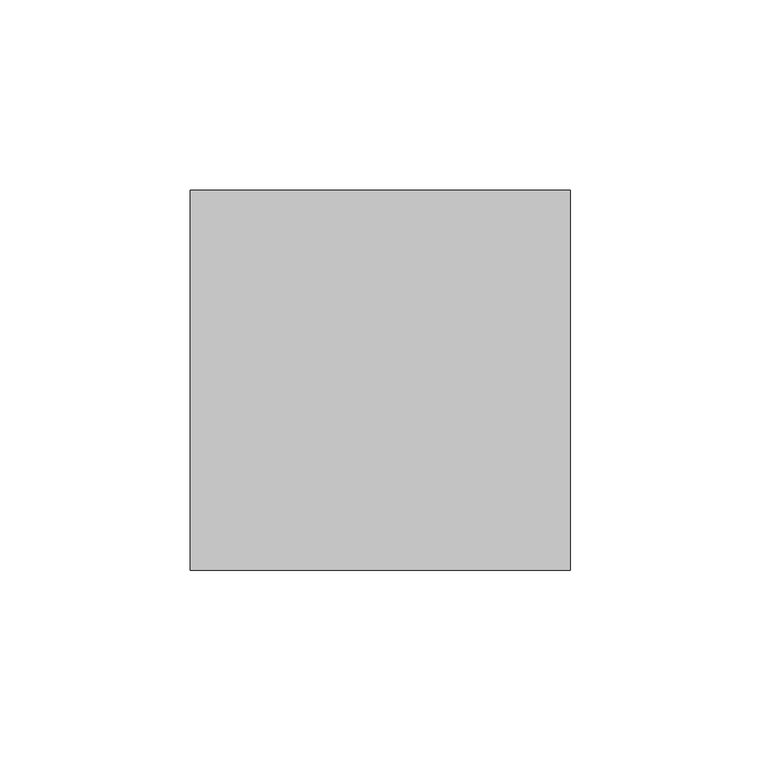
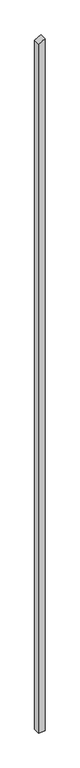
"""IFC4 building model written with IfcOpenShell, lengths in millimetres: column geometry, Holzstütze 159706 : Holzstütze 159706."""

import ifcopenshell
import ifcopenshell.guid

model = None  # the IFC model being written
_history = None  # IfcOwnerHistory: only IFC2X3 demands one
_inside = {}  # id of a spatial element -> (the spatial element, [elements in it])
_under = {}  # id of a project, library or spatial element -> (it, [spatial elements below it])
_declared = {}  # id of a project -> (the project, [libraries it declares])
_typed = {}  # id of a type object -> (the type object, [elements of that type])
_made_of = {}  # id of a material, layer set ... -> (it, [elements and type objects made of it])


def new_model(schema):
    """Start an empty IFC model of exactly this schema.

    Asked for "IFC4X3", IfcOpenShell would pick the latest addendum, in which some entities
    have other attributes; the version numbers below select the first issue.
    IFC2X3 requires an IfcOwnerHistory on every rooted entity: one is made here for all.
    """
    global model, _history
    if schema == "IFC4X3":
        model = ifcopenshell.file(schema_version=(4, 3, 0, 0))
    else:
        model = ifcopenshell.file(schema=schema)
    _inside.clear()
    _under.clear()
    _declared.clear()
    _typed.clear()
    _made_of.clear()
    _history = None
    if model.schema == "IFC2X3":
        org = make("IfcOrganization", Name="unknown")
        user = make(
            "IfcPersonAndOrganization",
            ThePerson=make("IfcPerson", FamilyName="unknown"),
            TheOrganization=org,
        )
        app = make(
            "IfcApplication",
            ApplicationDeveloper=org,
            Version="unknown",
            ApplicationFullName="unknown",
            ApplicationIdentifier="unknown",
        )
        _history = make(
            "IfcOwnerHistory",
            OwningUser=user,
            OwningApplication=app,
            ChangeAction="ADDED",
            CreationDate=0,
        )
    return model


def make(cls, **values):
    """One entity of the class cls with the attributes given. An attribute that is None is left unset."""
    return model.create_entity(
        cls, **{name: value for name, value in values.items() if value is not None}
    )


def rooted(cls, **values):
    """An entity with a GlobalId (a new one), such as an element, a storey or a relation."""
    return make(cls, GlobalId=ifcopenshell.guid.new(), OwnerHistory=_history, **values)


def si_unit(unit_type, name, prefix=None):
    """IfcSIUnit, for example si_unit("LENGTHUNIT", "METRE", prefix="MILLI")."""
    return make("IfcSIUnit", UnitType=unit_type, Prefix=prefix, Name=name)


def assignment(units):
    """IfcUnitAssignment: the units of a project."""
    return None if units is None else make("IfcUnitAssignment", Units=units)


def point(xyz):
    """IfcCartesianPoint."""
    return None if xyz is None else make("IfcCartesianPoint", Coordinates=xyz)


def direction(xyz):
    """IfcDirection."""
    return None if xyz is None else make("IfcDirection", DirectionRatios=xyz)


def frame(location, z_axis=None, x_axis=None):
    """IfcAxis2Placement3D, a coordinate frame: its origin and axes. An axis left out is left unset."""
    return make(
        "IfcAxis2Placement3D",
        Location=point(location),
        Axis=direction(z_axis),
        RefDirection=direction(x_axis),
    )


def origin():
    """The frame at (0, 0, 0) with its axes left unset."""
    return frame((0.0, 0.0, 0.0))


def place(relative_to, where):
    """IfcLocalPlacement: puts the frame where relative to a parent placement (None: the world)."""
    return make(
        "IfcLocalPlacement", PlacementRelTo=relative_to, RelativePlacement=where
    )


def context(
    kind, dimensions, precision=None, world=None, true_north=None, identifier=None
):
    """IfcGeometricRepresentationContext, for example the 3D "Model" context."""
    return make(
        "IfcGeometricRepresentationContext",
        ContextIdentifier=identifier,
        ContextType=kind,
        CoordinateSpaceDimension=dimensions,
        Precision=precision,
        WorldCoordinateSystem=world,
        TrueNorth=true_north,
    )


def project(units=None, contexts=None):
    """IfcProject with its units and contexts."""
    return rooted(
        "IfcProject",
        Name="project",
        RepresentationContexts=contexts,
        UnitsInContext=assignment(units),
    )


def spatial(cls, under=None, at=None, **own):
    """A site, building, storey or space (cls), placed at a placement, below another one or the project."""
    s = rooted(cls, ObjectPlacement=at, **own)
    if under is not None:
        _under.setdefault(under.id(), (under, []))[1].append(s)
    return s


def polyline(points):
    """IfcPolyline through the points."""
    return make("IfcPolyline", Points=[point(p) for p in points])


def outline(outer, holes=None, kind="AREA"):
    """IfcArbitraryClosedProfileDef: a profile drawn as a closed curve; with holes, ...WithVoids."""
    if holes is None:
        return make("IfcArbitraryClosedProfileDef", ProfileType=kind, OuterCurve=outer)
    return make(
        "IfcArbitraryProfileDefWithVoids",
        ProfileType=kind,
        OuterCurve=outer,
        InnerCurves=holes,
    )


def extrude(swept, where, along, depth):
    """IfcExtrudedAreaSolid: the profile swept, set in the frame where, extruded along a direction by depth."""
    return make(
        "IfcExtrudedAreaSolid",
        SweptArea=swept,
        Position=where,
        ExtrudedDirection=direction(along),
        Depth=depth,
    )


def shape(context_of_items, identifier, shape_type, items):
    """IfcShapeRepresentation: the items that make up one representation, for example the "Body"."""
    return make(
        "IfcShapeRepresentation",
        ContextOfItems=context_of_items,
        RepresentationIdentifier=identifier,
        RepresentationType=shape_type,
        Items=items,
    )


def source(mapping_origin, context_of_items, identifier, shape_type, items):
    """IfcRepresentationMap: a shape defined once, which mapped items show again and again."""
    return make(
        "IfcRepresentationMap",
        MappingOrigin=mapping_origin,
        MappedRepresentation=shape(context_of_items, identifier, shape_type, items),
    )


def transform(
    local_origin,
    x_axis=None,
    y_axis=None,
    z_axis=None,
    scale=None,
    scale2=None,
    scale3=None,
    uniform=True,
):
    """IfcCartesianTransformationOperator3D, or its non-uniform kind. x_axis, y_axis, z_axis: its Axis1, 2, 3."""
    if uniform:
        return make(
            "IfcCartesianTransformationOperator3D",
            Axis1=direction(x_axis),
            Axis2=direction(y_axis),
            LocalOrigin=point(local_origin),
            Scale=scale,
            Axis3=direction(z_axis),
        )
    return make(
        "IfcCartesianTransformationOperator3DnonUniform",
        Axis1=direction(x_axis),
        Axis2=direction(y_axis),
        LocalOrigin=point(local_origin),
        Scale=scale,
        Axis3=direction(z_axis),
        Scale2=scale2,
        Scale3=scale3,
    )


def mapped(mapping_source, mapping_target):
    """IfcMappedItem: shows the shape of a source again, moved by a transform."""
    return make(
        "IfcMappedItem", MappingSource=mapping_source, MappingTarget=mapping_target
    )


def made_of(thing, what):
    """Note that an element or type object is made of a material, layer set ...; save() writes the relation."""
    if what is not None:
        _made_of.setdefault(what.id(), (what, []))[1].append(thing)
    return thing


def element(
    cls,
    number,
    at=None,
    inside=None,
    cuts=None,
    type_object=None,
    material=None,
    context=None,
    identifier="Body",
    shape_type=None,
    held_by="IfcProductDefinitionShape",
    body=None,
    shapes=None,
    **own,
):
    """One element of the class cls, such as IfcWall. Its Tag is "e" and its number.

    at: its placement. inside: the storey or other place that contains it. cuts: it is an
    opening in that element (IfcRelVoidsElement). A single representation is given by context,
    identifier, shape_type and body (its items); several are given by shapes. held_by: the class
    of the entity that holds the representations. save() writes the other relations.
    """
    e = rooted(cls, Tag="e%d" % number, ObjectPlacement=at, **own)
    if body is not None:
        shapes = [shape(context, identifier, shape_type, body)]
    if shapes is not None:
        e.Representation = make(held_by, Representations=shapes)
    if inside is not None:
        _inside.setdefault(inside.id(), (inside, []))[1].append(e)
    if cuts is not None:
        rooted(
            "IfcRelVoidsElement", RelatingBuildingElement=cuts, RelatedOpeningElement=e
        )
    if type_object is not None:
        _typed.setdefault(type_object.id(), (type_object, []))[1].append(e)
    return made_of(e, material)


def aggregate(whole, parts):
    """IfcRelAggregates: a whole, such as a stair, and the parts it consists of."""
    return rooted("IfcRelAggregates", RelatingObject=whole, RelatedObjects=parts)


def save(model, path):
    """Write the relations noted so far, then the file.

    IfcRelAggregates (storeys below a building ...), IfcRelContainedInSpatialStructure (elements
    in a storey), IfcRelDefinesByType, IfcRelAssociatesMaterial and IfcRelDeclares: one each for
    every whole, place, type object, material and project.
    """
    for whole, parts in _under.values():
        aggregate(whole, parts)
    for where, things in _inside.values():
        rooted(
            "IfcRelContainedInSpatialStructure",
            RelatedElements=things,
            RelatingStructure=where,
        )
    for kind, things in _typed.values():
        rooted("IfcRelDefinesByType", RelatedObjects=things, RelatingType=kind)
    for what, things in _made_of.values():
        rooted("IfcRelAssociatesMaterial", RelatedObjects=things, RelatingMaterial=what)
    for by, libraries in _declared.values():
        rooted("IfcRelDeclares", RelatingContext=by, RelatedDefinitions=libraries)
    model.write(path)


def column_0947067b(model_context):
    return source(origin(), model_context, "Body", "SweptSolid", [
        extrude(outline(polyline([(-500.0, 165627.7593015), (-500.0, 165727.7593015), (10641.011365, 165727.7593015), (10590.0588201, 165627.7593015), (-500.0, 165627.7593015)])), frame((0.0, 26981.9343946, 0.0), z_axis=(0.0, 1.0, 0.0), x_axis=(0.0, 0.0, 1.0)), (0.0, 0.0, 1.0), 100.0),
    ])


if __name__ == "__main__":
    model = new_model("IFC4")
    model_context = context("Model", 3, world=origin())
    ifc_project = project(units=[si_unit("LENGTHUNIT", "METRE", prefix="MILLI")], contexts=[model_context])
    site = spatial("IfcSite", under=ifc_project)
    building = spatial("IfcBuilding", under=site)
    placement = place(None, origin())
    column_shape = column_0947067b(model_context)
    element("IfcColumn", 1, ObjectType="Holzstütze 159706 : Holzstütze 159706", at=placement, inside=building, context=model_context, shape_type="MappedRepresentation", body=[
        mapped(column_shape, transform((0.0, 0.0, 0.0), x_axis=(1.0, 0.0, 0.0), y_axis=(0.0, 1.0, 0.0), z_axis=(0.0, 0.0, 1.0))),
    ])
    save(model, "model.ifc")

# Revit data of these elements
# Type "Holzstütze 159706 : Holzstütze 159706"
#   Abrechnungsart = "m"
#   Allright_Bauteil_ID = "0152St 0000143522"
#   Bezeichnung = "Holzstütze"
#   Codetext = "ST-HOLZ\\"
#   Gewerk = "Zimmer- und Holzbauarbeiten"
#   Material = "Holz"
#   Objektname = "Stütze"
#   NameOverride = "Holzstütze"
#   Reference = "Holzstütze"
#   Status = "NEW"
#   ThermalTransmittance = 0.0000 BTU/(h·ft²·°F)
#   Roll = 0.00°
#   Slope = 0.00°
#   2D Interaktion = yes
#   IsExternal = yes
#   LoadBearing = yes
# Element 1 (IfcColumn, "Holzstütze 159706 : Holzstütze 159706")
#   Materials on its faces: "holzschalung"
# Materials
#   "holzschalung": class "Unassigned", colour RGB 128 128 128, transparency 0
